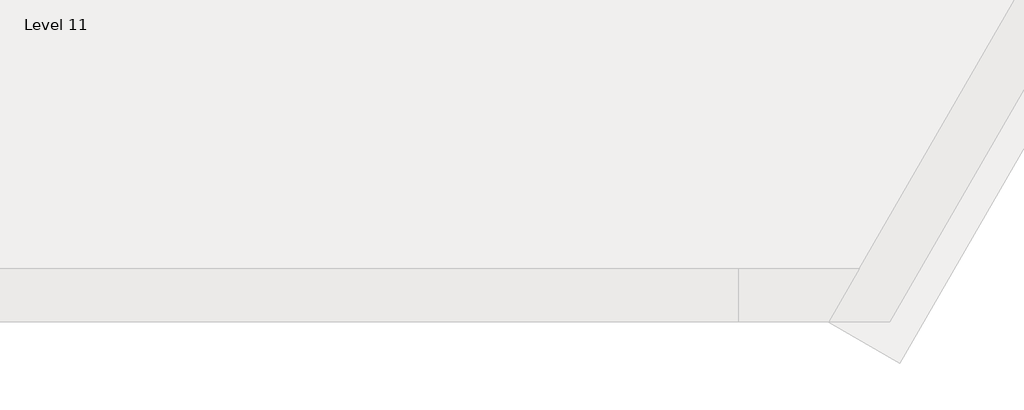
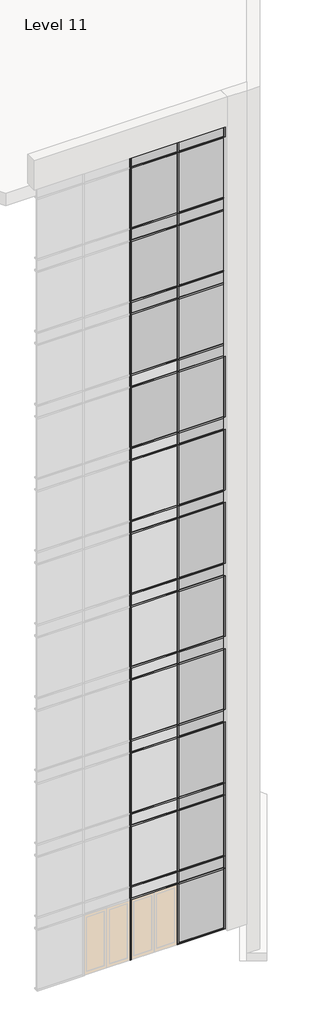
# One storey, part 3 of 6: 100 members, 29 plates.
# Revit data of these elements (continued)
# Type "System Panel : Glazed" (continued)
#   Construction Type Id = "GSP4R"
#   Analytic Construction = "1/8 in Pilkington single glazing"
#   Visual Light Transmittance = 0.9
#   Solar Heat Gain Coefficient = 0.86
#   Heat Transfer Coefficient (U) = 6.7069 W/(m²·K)
# Elements 1, 2, 3, 4, 5, 6, 7, 8, 9, 10, 11, 12, 13, 14, 15, 16, 17, 18, 19, 20, 21, 22, 23, 24, 25, 26, 27, 28, 29, 30, 31, 32, 33, 34, 35, 36, 37, 38, 39, 40, 41, 42, 43, 44, 45, 46, 47, 48, 49, 50, 51, 52, 53, 54, 55, 56, 57, 58, 59, 60, 61, 62, 63, 64, 65, 66, 67, 68, 69, 70, 71, 72, 73, 74, 75, 76, 77, 78, 79, 80, 81, 82, 83, 84, 85, 86, 87, 88, 89, 90, 91, 92, 93, 94, 95, 96, 97, 98, 99, 100 (IfcMember, "Rectangular Mullion : 50x150mm")
#   Phase Created = New Construction
#   Materials on its faces: "Aluminium"
# Elements 101, 102, 103, 104, 105, 106, 107, 108, 109, 110, 111, 112, 113, 114, 115, 116, 117, 118, 119, 120, 121, 122, 123, 124, 125, 126, 127, 128, 129 (IfcPlate, "System Panel : Glazed")
#   Phase Created = New Construction
#   Materials on its faces: "Glass"
# Materials
#   "Aluminium": class "Metal", colour RGB 247 247 247, transparency 0, Description = "Aluminium 6061", Cost = 0
#   "Glass": class "Glass", colour RGB 0 128 192, transparency 0.9, Description = "Soda Lime Glass", Cost = 0
